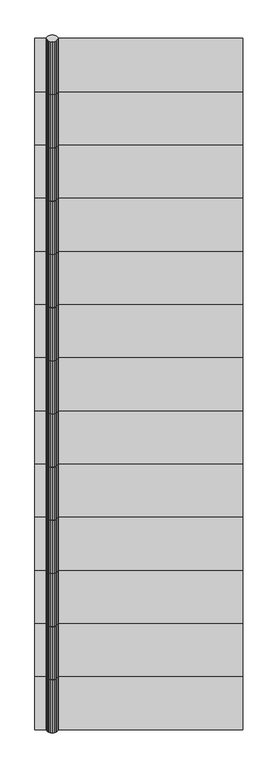
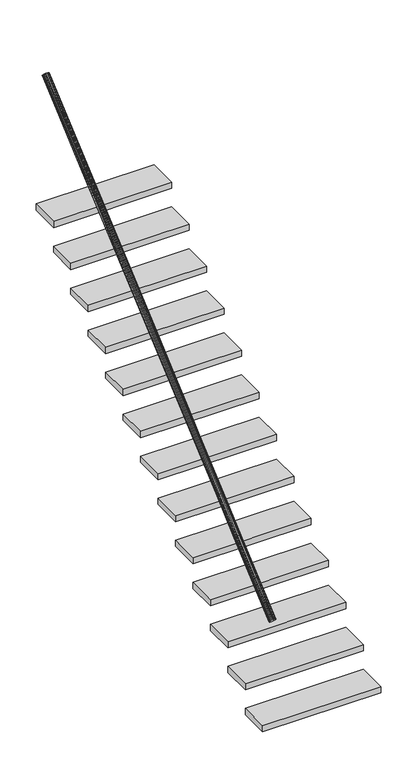
"""IFC4 building model written with IfcOpenShell, lengths in millimetres: stair geometry, 0_3d_modell."""

from ifc_helpers import new_model, si_unit, frame, origin, origin_with_axes, place, context, project, spatial, polyline, outline, extrude, source, transform, mapped, element, save


def stair_1067d48f(model_context):
    return source(origin(), model_context, "Body", "SweptSolid", [
        extrude(outline(polyline([(1.2235871, -7.065663), (0.0, 0.0), (1.2235871, 7.0656631), (4.7745751, 13.4396897), (10.3053687, 18.498146), (17.2745751, 21.7458748), (25.0, 22.8649659), (32.7254249, 21.7458748), (39.6946313, 18.498146), (45.2254249, 13.4396897), (48.7764129, 7.0656631), (50.0, 0.0), (48.7764129, -7.065663), (45.2254249, -13.4396898), (39.6946313, -18.498146), (32.7254249, -21.7458748), (25.0, -22.8649659), (17.2745751, -21.7458748), (10.3053687, -18.498146), (4.7745751, -13.4396898), (1.2235871, -7.065663)])), frame((50.0, 704.9421971, 1465.2735223), z_axis=(0.0, 0.7569287102857122, 0.6534974579485435), x_axis=(1.0, 0.0, 0.0)), (0.0, 0.0, 1.0), 303.8595272),
        extrude(outline(polyline([(1.2235871, -7.0656631), (0.0, 0.0), (1.2235871, 7.0656631), (4.7745751, 13.4396897), (10.3053687, 18.498146), (17.2745751, 21.7458748), (25.0, 22.8649659), (32.7254249, 21.7458748), (39.6946313, 18.498146), (45.2254249, 13.4396897), (48.7764129, 7.0656631), (50.0, 0.0), (48.7764129, -7.0656631), (45.2254249, -13.4396898), (39.6946313, -18.4981461), (32.7254249, -21.7458748), (25.0, -22.8649659), (17.2745751, -21.7458748), (10.3053687, -18.4981461), (4.7745751, -13.4396898), (1.2235871, -7.0656631)])), frame((50.0, 2084.9421971, 2656.7020937), z_axis=(0.0, 0.7569287102856974, 0.6534974579485607), x_axis=(1.0, 0.0, 0.0)), (0.0, 0.0, 1.0), 303.8595272),
        extrude(outline(polyline([(1.2235871, -7.065663), (0.0, 0.0), (1.2235871, 7.0656631), (4.7745751, 13.4396898), (10.3053687, 18.498146), (17.2745751, 21.7458748), (25.0, 22.8649659), (32.7254249, 21.7458748), (39.6946313, 18.498146), (45.2254249, 13.4396898), (48.7764129, 7.0656631), (50.0, 0.0), (48.7764129, -7.065663), (45.2254249, -13.4396897), (39.6946313, -18.498146), (32.7254249, -21.7458748), (25.0, -22.8649659), (17.2745751, -21.7458748), (10.3053687, -18.498146), (4.7745751, -13.4396897), (1.2235871, -7.065663)])), frame((50.0, 2544.9421971, 3053.8449509), z_axis=(0.0, 0.756928710285712, 0.6534974579485439), x_axis=(1.0, 0.0, 0.0)), (0.0, 0.0, 1.0), 303.8595272),
        extrude(outline(polyline([(900.0, 934.9421971), (0.0, 934.9421971), (0.0, 1164.9421971), (900.0, 1164.9421971), (900.0, 934.9421971)])), frame((0.0, 0.0, 794.2857143), z_axis=(0.0, 0.0, 1.0), x_axis=(1.0, 0.0, 0.0)), (0.0, 0.0, 1.0), 50.0),
        extrude(outline(polyline([(1.2235871, -7.065663), (0.0, 0.0), (1.2235871, 7.0656631), (4.7745751, 13.4396897), (10.3053687, 18.498146), (17.2745751, 21.7458748), (25.0, 22.8649659), (32.7254249, 21.7458748), (39.6946313, 18.498146), (45.2254249, 13.4396897), (48.7764129, 7.0656631), (50.0, 0.0), (48.7764129, -7.065663), (45.2254249, -13.4396897), (39.6946313, -18.498146), (32.7254249, -21.7458748), (25.0, -22.8649659), (17.2745751, -21.7458748), (10.3053687, -18.498146), (4.7745751, -13.4396897), (1.2235871, -7.065663)])), frame((50.0, 1624.9421971, 2259.5592366), z_axis=(0.0, 0.7569287102856798, 0.6534974579485812), x_axis=(1.0, 0.0, 0.0)), (0.0, 0.0, 1.0), 303.8595272),
        extrude(outline(polyline([(900.0, 704.9421971), (0.0, 704.9421971), (0.0, 934.9421971), (900.0, 934.9421971), (900.0, 704.9421971)])), frame((0.0, 0.0, 595.7142857), z_axis=(0.0, 0.0, 1.0), x_axis=(1.0, 0.0, 0.0)), (0.0, 0.0, 1.0), 50.0),
        extrude(outline(polyline([(1.2235871, -7.065663), (0.0, 0.0), (1.2235871, 7.0656631), (4.7745751, 13.4396897), (10.3053687, 18.498146), (17.2745751, 21.7458748), (25.0, 22.8649659), (32.7254249, 21.7458748), (39.6946313, 18.498146), (45.2254249, 13.4396897), (48.7764129, 7.0656631), (50.0, 0.0), (48.7764129, -7.065663), (45.2254249, -13.4396897), (39.6946313, -18.498146), (32.7254249, -21.7458748), (25.0, -22.8649659), (17.2745751, -21.7458748), (10.3053687, -18.498146), (4.7745751, -13.4396897), (1.2235871, -7.065663)])), frame((50.0, 14.9421971, 869.5592366), z_axis=(0.0, 0.7569287102857073, 0.6534974579485493), x_axis=(1.0, 0.0, 0.0)), (0.0, 0.0, 1.0), 303.8595272),
        extrude(outline(polyline([(1.2235871, -7.065663), (0.0, 0.0), (1.2235871, 7.0656631), (4.7745751, 13.4396898), (10.3053687, 18.498146), (17.2745751, 21.7458748), (25.0, 22.8649659), (32.7254249, 21.7458748), (39.6946313, 18.498146), (45.2254249, 13.4396898), (48.7764129, 7.0656631), (50.0, 0.0), (48.7764129, -7.065663), (45.2254249, -13.4396897), (39.6946313, -18.498146), (32.7254249, -21.7458748), (25.0, -22.8649659), (17.2745751, -21.7458748), (10.3053687, -18.498146), (4.7745751, -13.4396897), (1.2235871, -7.065663)])), frame((50.0, 244.9421971, 1068.1306652), z_axis=(0.0, 0.7569287102856902, 0.6534974579485691), x_axis=(1.0, 0.0, 0.0)), (0.0, 0.0, 1.0), 303.8595272),
        extrude(outline(polyline([(900.0, 1164.9421971), (0.0, 1164.9421971), (0.0, 1394.9421971), (900.0, 1394.9421971), (900.0, 1164.9421971)])), frame((0.0, 0.0, 992.8571429), z_axis=(0.0, 0.0, 1.0), x_axis=(1.0, 0.0, 0.0)), (0.0, 0.0, 1.0), 50.0),
        extrude(outline(polyline([(900.0, 14.9421971), (0.0, 14.9421971), (0.0, 244.9421971), (900.0, 244.9421971), (900.0, 14.9421971)])), origin_with_axes(), (0.0, 0.0, 1.0), 50.0),
        extrude(outline(polyline([(900.0, 1854.9421971), (0.0, 1854.9421971), (0.0, 2084.9421971), (900.0, 2084.9421971), (900.0, 1854.9421971)])), frame((0.0, 0.0, 1588.5714286), z_axis=(0.0, 0.0, 1.0), x_axis=(1.0, 0.0, 0.0)), (0.0, 0.0, 1.0), 50.0),
        extrude(outline(polyline([(900.0, 244.9421971), (0.0, 244.9421971), (0.0, 474.9421971), (900.0, 474.9421971), (900.0, 244.9421971)])), frame((0.0, 0.0, 198.5714286), z_axis=(0.0, 0.0, 1.0), x_axis=(1.0, 0.0, 0.0)), (0.0, 0.0, 1.0), 50.0),
        extrude(outline(polyline([(1.2235871, -7.065663), (0.0, 0.0), (1.2235871, 7.0656631), (4.7745751, 13.4396898), (10.3053687, 18.498146), (17.2745751, 21.7458748), (25.0, 22.8649659), (32.7254249, 21.7458748), (39.6946313, 18.498146), (45.2254249, 13.4396898), (48.7764129, 7.0656631), (50.0, 0.0), (48.7764129, -7.065663), (45.2254249, -13.4396897), (39.6946313, -18.498146), (32.7254249, -21.7458748), (25.0, -22.8649659), (17.2745751, -21.7458748), (10.3053687, -18.498146), (4.7745751, -13.4396897), (1.2235871, -7.065663)])), frame((50.0, 934.9421971, 1663.8449509), z_axis=(0.0, 0.7569287102857108, 0.6534974579485451), x_axis=(1.0, 0.0, 0.0)), (0.0, 0.0, 1.0), 303.8595272),
        extrude(outline(polyline([(1.2235871, -7.065663), (0.0, 0.0), (1.2235871, 7.0656631), (4.7745751, 13.4396898), (10.3053687, 18.498146), (17.2745751, 21.7458748), (25.0, 22.8649659), (32.7254249, 21.7458748), (39.6946313, 18.498146), (45.2254249, 13.4396898), (48.7764129, 7.0656631), (50.0, 0.0), (48.7764129, -7.065663), (45.2254249, -13.4396897), (39.6946313, -18.498146), (32.7254249, -21.7458748), (25.0, -22.8649659), (17.2745751, -21.7458748), (10.3053687, -18.498146), (4.7745751, -13.4396897), (1.2235871, -7.065663)])), frame((50.0, 2774.9421971, 3252.4163795), z_axis=(0.0, 0.7569287102857426, 0.6534974579485083), x_axis=(1.0, 0.0, 0.0)), (0.0, 0.0, 1.0), 303.8595272),
        extrude(outline(polyline([(900.0, 2084.9421971), (0.0, 2084.9421971), (0.0, 2314.9421971), (900.0, 2314.9421971), (900.0, 2084.9421971)])), frame((0.0, 0.0, 1787.1428571), z_axis=(0.0, 0.0, 1.0), x_axis=(1.0, 0.0, 0.0)), (0.0, 0.0, 1.0), 50.0),
        extrude(outline(polyline([(1.2235871, -7.065663), (0.0, 0.0), (1.2235871, 7.0656631), (4.7745751, 13.4396898), (10.3053687, 18.498146), (17.2745751, 21.7458748), (25.0, 22.8649659), (32.7254249, 21.7458748), (39.6946313, 18.498146), (45.2254249, 13.4396898), (48.7764129, 7.0656631), (50.0, 0.0), (48.7764129, -7.065663), (45.2254249, -13.4396897), (39.6946313, -18.498146), (32.7254249, -21.7458748), (25.0, -22.8649659), (17.2745751, -21.7458748), (10.3053687, -18.498146), (4.7745751, -13.4396897), (1.2235871, -7.065663)])), frame((50.0, 1164.9421971, 1862.4163795), z_axis=(0.0, 0.7569287102857027, 0.6534974579485544), x_axis=(1.0, 0.0, 0.0)), (0.0, 0.0, 1.0), 303.8595272),
        extrude(outline(polyline([(900.0, 2774.9421971), (0.0, 2774.9421971), (0.0, 3004.9421971), (900.0, 3004.9421971), (900.0, 2774.9421971)])), frame((0.0, 0.0, 2382.8571429), z_axis=(0.0, 0.0, 1.0), x_axis=(1.0, 0.0, 0.0)), (0.0, 0.0, 1.0), 50.0),
        extrude(outline(polyline([(900.0, 2314.9421971), (0.0, 2314.9421971), (0.0, 2544.9421971), (900.0, 2544.9421971), (900.0, 2314.9421971)])), frame((0.0, 0.0, 1985.7142857), z_axis=(0.0, 0.0, 1.0), x_axis=(1.0, 0.0, 0.0)), (0.0, 0.0, 1.0), 50.0),
        extrude(outline(polyline([(1.2235871, -7.0656631), (0.0, 0.0), (1.2235871, 7.0656631), (4.7745751, 13.4396897), (10.3053687, 18.498146), (17.2745751, 21.7458748), (25.0, 22.8649659), (32.7254249, 21.7458748), (39.6946313, 18.498146), (45.2254249, 13.4396897), (48.7764129, 7.0656631), (50.0, 0.0), (48.7764129, -7.0656631), (45.2254249, -13.4396898), (39.6946313, -18.498146), (32.7254249, -21.7458748), (25.0, -22.8649659), (17.2745751, -21.7458748), (10.3053687, -18.498146), (4.7745751, -13.4396898), (1.2235871, -7.0656631)])), frame((50.0, 1394.9421971, 2060.987808), z_axis=(0.0, 0.7569287102856966, 0.6534974579485615), x_axis=(1.0, 0.0, 0.0)), (0.0, 0.0, 1.0), 303.8595272),
        extrude(outline(polyline([(900.0, 2544.9421971), (0.0, 2544.9421971), (0.0, 2774.9421971), (900.0, 2774.9421971), (900.0, 2544.9421971)])), frame((0.0, 0.0, 2184.2857143), z_axis=(0.0, 0.0, 1.0), x_axis=(1.0, 0.0, 0.0)), (0.0, 0.0, 1.0), 50.0),
        extrude(outline(polyline([(900.0, 474.9421971), (0.0, 474.9421971), (0.0, 704.9421971), (900.0, 704.9421971), (900.0, 474.9421971)])), frame((0.0, 0.0, 397.1428571), z_axis=(0.0, 0.0, 1.0), x_axis=(1.0, 0.0, 0.0)), (0.0, 0.0, 1.0), 50.0),
        extrude(outline(polyline([(900.0, 1394.9421971), (0.0, 1394.9421971), (0.0, 1624.9421971), (900.0, 1624.9421971), (900.0, 1394.9421971)])), frame((0.0, 0.0, 1191.4285714), z_axis=(0.0, 0.0, 1.0), x_axis=(1.0, 0.0, 0.0)), (0.0, 0.0, 1.0), 50.0),
        extrude(outline(polyline([(1.2235871, -7.065663), (0.0, 0.0), (1.2235871, 7.0656631), (4.7745751, 13.4396898), (10.3053687, 18.498146), (17.2745751, 21.7458748), (25.0, 22.8649659), (32.7254249, 21.7458748), (39.6946313, 18.498146), (45.2254249, 13.4396898), (48.7764129, 7.0656631), (50.0, 0.0), (48.7764129, -7.065663), (45.2254249, -13.4396897), (39.6946313, -18.498146), (32.7254249, -21.7458748), (25.0, -22.8649659), (17.2745751, -21.7458748), (10.3053687, -18.498146), (4.7745751, -13.4396897), (1.2235871, -7.065663)])), frame((50.0, 1854.9421971, 2458.1306652), z_axis=(0.0, 0.7569287102857091, 0.6534974579485472), x_axis=(1.0, 0.0, 0.0)), (0.0, 0.0, 1.0), 303.8595272),
        extrude(outline(polyline([(900.0, 1624.9421971), (0.0, 1624.9421971), (0.0, 1854.9421971), (900.0, 1854.9421971), (900.0, 1624.9421971)])), frame((0.0, 0.0, 1390.0), z_axis=(0.0, 0.0, 1.0), x_axis=(1.0, 0.0, 0.0)), (0.0, 0.0, 1.0), 50.0),
        extrude(outline(polyline([(1.2235871, -7.065663), (0.0, 0.0), (1.2235871, 7.0656631), (4.7745751, 13.4396897), (10.3053687, 18.498146), (17.2745751, 21.7458748), (25.0, 22.8649659), (32.7254249, 21.7458748), (39.6946313, 18.498146), (45.2254249, 13.4396897), (48.7764129, 7.0656631), (50.0, 0.0), (48.7764129, -7.065663), (45.2254249, -13.4396898), (39.6946313, -18.498146), (32.7254249, -21.7458748), (25.0, -22.8649659), (17.2745751, -21.7458748), (10.3053687, -18.498146), (4.7745751, -13.4396898), (1.2235871, -7.065663)])), frame((50.0, 2314.9421971, 2855.2735223), z_axis=(0.0, 0.756928710285704, 0.653497457948553), x_axis=(1.0, 0.0, 0.0)), (0.0, 0.0, 1.0), 303.8595272),
        extrude(outline(polyline([(1.2235871, -7.0656631), (0.0, 0.0), (1.2235871, 7.0656631), (4.7745751, 13.4396897), (10.3053687, 18.498146), (17.2745751, 21.7458748), (25.0, 22.8649659), (32.7254249, 21.7458748), (39.6946313, 18.498146), (45.2254249, 13.4396897), (48.7764129, 7.0656631), (50.0, 0.0), (48.7764129, -7.0656631), (45.2254249, -13.4396898), (39.6946313, -18.4981461), (32.7254249, -21.7458748), (25.0, -22.8649659), (17.2745751, -21.7458748), (10.3053687, -18.4981461), (4.7745751, -13.4396898), (1.2235871, -7.0656631)])), frame((50.0, 474.9421971, 1266.7020937), z_axis=(0.0, 0.7569287102857101, 0.653497457948546), x_axis=(1.0, 0.0, 0.0)), (0.0, 0.0, 1.0), 303.8595272),
    ])


if __name__ == "__main__":
    model = new_model("IFC4")
    model_context = context("Model", 3, world=origin())
    ifc_project = project(units=[si_unit("LENGTHUNIT", "METRE", prefix="MILLI")], contexts=[model_context])
    site = spatial("IfcSite", under=ifc_project)
    building = spatial("IfcBuilding", under=site)
    placement = place(None, origin())
    stair_shape = stair_1067d48f(model_context)
    element("IfcStair", 1, ObjectType="0_3d_modell", at=placement, inside=building, context=model_context, shape_type="MappedRepresentation", body=[
        mapped(stair_shape, transform((0.0, 0.0, 0.0), x_axis=(1.0, 0.0, 0.0), y_axis=(0.0, 1.0, 0.0), z_axis=(0.0, 0.0, 1.0))),
    ])
    save(model, "model.ifc")

# Revit data of these elements
# Element 1 (IfcStair, "0_3d_modell")
#   Materials on its faces: "*1", "weiss"
# Materials
#   "*1": class "Unassigned", colour RGB 175 175 175, transparency 0
#   "weiss": class "Unassigned", colour RGB 255 255 255, transparency 0
